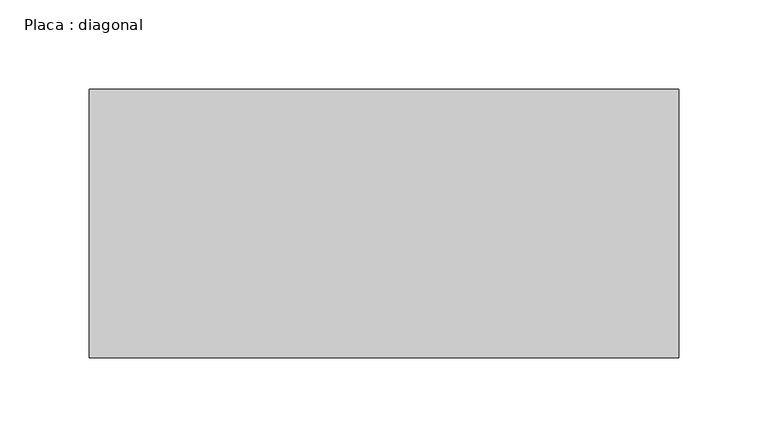
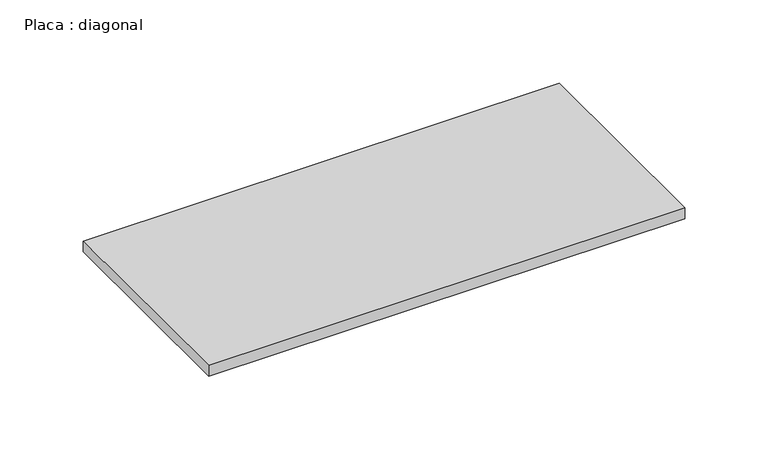
"""IFC4 building model written with IfcOpenShell, lengths in millimetres: beam geometry, Placa : diagonal."""

from ifc_helpers import new_model, si_unit, frame, origin, place, context, project, spatial, polyline, outline, extrude, source, transform, mapped, element, save


def placa_diagonal_77673082(model_context):
    return source(origin(), model_context, "Body", "SweptSolid", [
        extrude(outline(polyline([(164.7911476, 75.0), (164.7911476, -75.0), (-164.7911476, -75.0), (-164.7911476, 75.0), (164.7911476, 75.0)])), frame((0.0, 0.0, -4.0), z_axis=(0.0, 0.0, 1.0), x_axis=(1.0, 0.0, 0.0)), (0.0, 0.0, 1.0), 8.0),
    ])


if __name__ == "__main__":
    model = new_model("IFC4")
    model_context = context("Model", 3, world=origin())
    ifc_project = project(units=[si_unit("LENGTHUNIT", "METRE", prefix="MILLI")], contexts=[model_context])
    site = spatial("IfcSite", under=ifc_project)
    building = spatial("IfcBuilding", under=site)
    placement = place(None, origin())
    placa_diagonal_shape = placa_diagonal_77673082(model_context)
    element("IfcBeam", 1, ObjectType="Placa : diagonal", at=placement, inside=building, context=model_context, shape_type="MappedRepresentation", body=[
        mapped(placa_diagonal_shape, transform((0.0, 0.0, 0.0), x_axis=(1.0, 0.0, 0.0), y_axis=(0.0, 1.0, 0.0), z_axis=(0.0, 0.0, 1.0))),
    ])
    save(model, "model.ifc")

# Revit data of these elements
# Type "Placa : diagonal"
#   W = 0
#   Length [instance default] = 1.50 m
#   b = 0.15 m
#   d = 0.008 m
#   A = 0 m²
#   Structural Material [instance default] = Aço, 45-345
# Element 1 (IfcBeam, "Placa : diagonal")
#   Materials on its faces: "Aço, 45-345"
# Materials
#   "Aço, 45-345": class "Metal", colour RGB 247 247 247, transparency 0, Description = "Aço 345 MPa", Cost = 0
